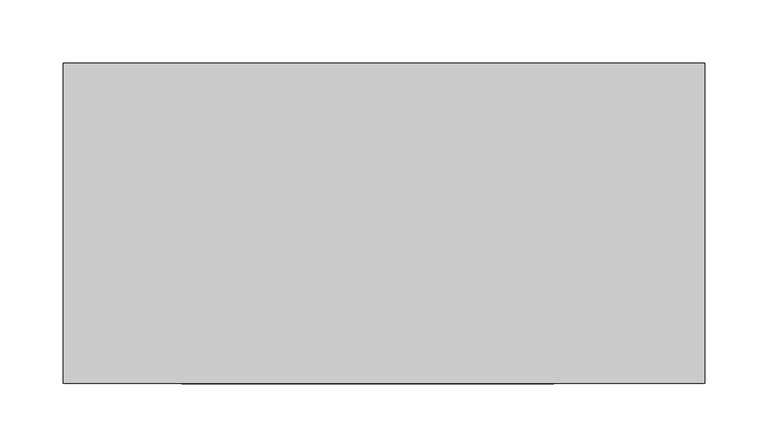
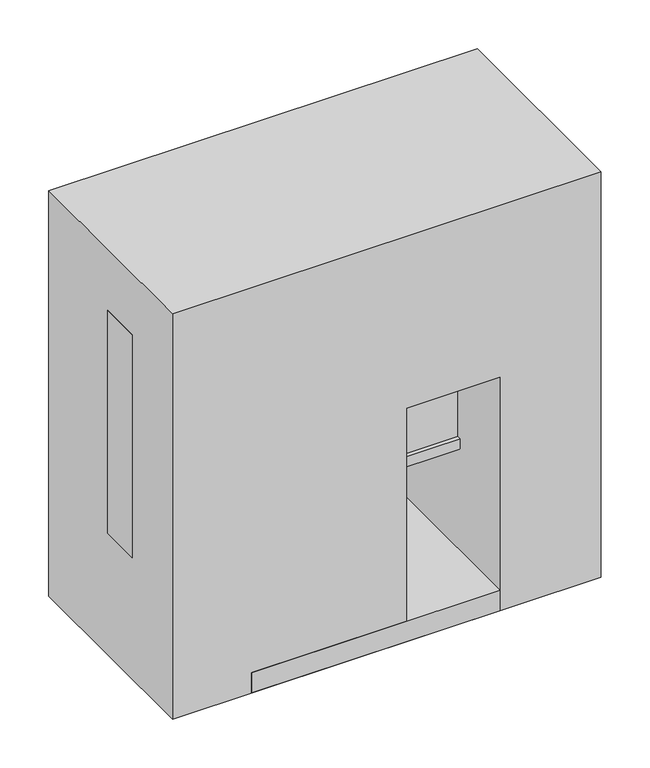
"""IFC4 building model written with IfcOpenShell, lengths in millimetres: proxy geometry, X4110 - Console, PACS, Remote View, 512 X 512, 1 Monitor : X4110 - Console, PACS, Remote View, 512 X 512, 1 Monitor."""

import ifcopenshell
import ifcopenshell.guid

model = None  # the IFC model being written
_history = None  # IfcOwnerHistory: only IFC2X3 demands one
_inside = {}  # id of a spatial element -> (the spatial element, [elements in it])
_under = {}  # id of a project, library or spatial element -> (it, [spatial elements below it])
_declared = {}  # id of a project -> (the project, [libraries it declares])
_typed = {}  # id of a type object -> (the type object, [elements of that type])
_made_of = {}  # id of a material, layer set ... -> (it, [elements and type objects made of it])


def new_model(schema):
    """Start an empty IFC model of exactly this schema.

    Asked for "IFC4X3", IfcOpenShell would pick the latest addendum, in which some entities
    have other attributes; the version numbers below select the first issue.
    IFC2X3 requires an IfcOwnerHistory on every rooted entity: one is made here for all.
    """
    global model, _history
    if schema == "IFC4X3":
        model = ifcopenshell.file(schema_version=(4, 3, 0, 0))
    else:
        model = ifcopenshell.file(schema=schema)
    _inside.clear()
    _under.clear()
    _declared.clear()
    _typed.clear()
    _made_of.clear()
    _history = None
    if model.schema == "IFC2X3":
        org = make("IfcOrganization", Name="unknown")
        user = make(
            "IfcPersonAndOrganization",
            ThePerson=make("IfcPerson", FamilyName="unknown"),
            TheOrganization=org,
        )
        app = make(
            "IfcApplication",
            ApplicationDeveloper=org,
            Version="unknown",
            ApplicationFullName="unknown",
            ApplicationIdentifier="unknown",
        )
        _history = make(
            "IfcOwnerHistory",
            OwningUser=user,
            OwningApplication=app,
            ChangeAction="ADDED",
            CreationDate=0,
        )
    return model


def make(cls, **values):
    """One entity of the class cls with the attributes given. An attribute that is None is left unset."""
    return model.create_entity(
        cls, **{name: value for name, value in values.items() if value is not None}
    )


def rooted(cls, **values):
    """An entity with a GlobalId (a new one), such as an element, a storey or a relation."""
    return make(cls, GlobalId=ifcopenshell.guid.new(), OwnerHistory=_history, **values)


def si_unit(unit_type, name, prefix=None):
    """IfcSIUnit, for example si_unit("LENGTHUNIT", "METRE", prefix="MILLI")."""
    return make("IfcSIUnit", UnitType=unit_type, Prefix=prefix, Name=name)


def assignment(units):
    """IfcUnitAssignment: the units of a project."""
    return None if units is None else make("IfcUnitAssignment", Units=units)


def point(xyz):
    """IfcCartesianPoint."""
    return None if xyz is None else make("IfcCartesianPoint", Coordinates=xyz)


def direction(xyz):
    """IfcDirection."""
    return None if xyz is None else make("IfcDirection", DirectionRatios=xyz)


def frame(location, z_axis=None, x_axis=None):
    """IfcAxis2Placement3D, a coordinate frame: its origin and axes. An axis left out is left unset."""
    return make(
        "IfcAxis2Placement3D",
        Location=point(location),
        Axis=direction(z_axis),
        RefDirection=direction(x_axis),
    )


def origin():
    """The frame at (0, 0, 0) with its axes left unset."""
    return frame((0.0, 0.0, 0.0))


def place(relative_to, where):
    """IfcLocalPlacement: puts the frame where relative to a parent placement (None: the world)."""
    return make(
        "IfcLocalPlacement", PlacementRelTo=relative_to, RelativePlacement=where
    )


def context(
    kind, dimensions, precision=None, world=None, true_north=None, identifier=None
):
    """IfcGeometricRepresentationContext, for example the 3D "Model" context."""
    return make(
        "IfcGeometricRepresentationContext",
        ContextIdentifier=identifier,
        ContextType=kind,
        CoordinateSpaceDimension=dimensions,
        Precision=precision,
        WorldCoordinateSystem=world,
        TrueNorth=true_north,
    )


def project(units=None, contexts=None):
    """IfcProject with its units and contexts."""
    return rooted(
        "IfcProject",
        Name="project",
        RepresentationContexts=contexts,
        UnitsInContext=assignment(units),
    )


def spatial(cls, under=None, at=None, **own):
    """A site, building, storey or space (cls), placed at a placement, below another one or the project."""
    s = rooted(cls, ObjectPlacement=at, **own)
    if under is not None:
        _under.setdefault(under.id(), (under, []))[1].append(s)
    return s


def faces_of(points, faces, orient=None, outer=None):
    """IfcFace entities. A face is a list of loops; a loop is a list of indices into points, from 0.

    orient and outer hold one flag for each loop. By default every Orientation is true, the
    first loop of a face is its IfcFaceOuterBound and the others are IfcFaceBound.
    """
    made = []
    for i, loops in enumerate(faces):
        bounds = []
        for j, loop in enumerate(loops):
            is_outer = j == 0 if outer is None else outer[i][j]
            bounds.append(
                make(
                    "IfcFaceOuterBound" if is_outer else "IfcFaceBound",
                    Bound=make("IfcPolyLoop", Polygon=[points[k] for k in loop]),
                    Orientation=True if orient is None else orient[i][j],
                )
            )
        made.append(make("IfcFace", Bounds=bounds))
    return made


def faceted_brep(points, faces, orient=None, outer=None, voids=None):
    """IfcFacetedBrep: a solid bounded by flat faces; with voids (closed shells), ...WithVoids."""
    shared = [point(p) for p in points]
    hull = make("IfcClosedShell", CfsFaces=faces_of(shared, faces, orient, outer))
    if voids is None:
        return make("IfcFacetedBrep", Outer=hull)
    return make(
        "IfcFacetedBrepWithVoids",
        Outer=hull,
        Voids=[
            make(cls, CfsFaces=faces_of(shared, fs, o, b)) for cls, fs, o, b in voids
        ],
    )


def shape(context_of_items, identifier, shape_type, items):
    """IfcShapeRepresentation: the items that make up one representation, for example the "Body"."""
    return make(
        "IfcShapeRepresentation",
        ContextOfItems=context_of_items,
        RepresentationIdentifier=identifier,
        RepresentationType=shape_type,
        Items=items,
    )


def source(mapping_origin, context_of_items, identifier, shape_type, items):
    """IfcRepresentationMap: a shape defined once, which mapped items show again and again."""
    return make(
        "IfcRepresentationMap",
        MappingOrigin=mapping_origin,
        MappedRepresentation=shape(context_of_items, identifier, shape_type, items),
    )


def transform(
    local_origin,
    x_axis=None,
    y_axis=None,
    z_axis=None,
    scale=None,
    scale2=None,
    scale3=None,
    uniform=True,
):
    """IfcCartesianTransformationOperator3D, or its non-uniform kind. x_axis, y_axis, z_axis: its Axis1, 2, 3."""
    if uniform:
        return make(
            "IfcCartesianTransformationOperator3D",
            Axis1=direction(x_axis),
            Axis2=direction(y_axis),
            LocalOrigin=point(local_origin),
            Scale=scale,
            Axis3=direction(z_axis),
        )
    return make(
        "IfcCartesianTransformationOperator3DnonUniform",
        Axis1=direction(x_axis),
        Axis2=direction(y_axis),
        LocalOrigin=point(local_origin),
        Scale=scale,
        Axis3=direction(z_axis),
        Scale2=scale2,
        Scale3=scale3,
    )


def mapped(mapping_source, mapping_target):
    """IfcMappedItem: shows the shape of a source again, moved by a transform."""
    return make(
        "IfcMappedItem", MappingSource=mapping_source, MappingTarget=mapping_target
    )


def made_of(thing, what):
    """Note that an element or type object is made of a material, layer set ...; save() writes the relation."""
    if what is not None:
        _made_of.setdefault(what.id(), (what, []))[1].append(thing)
    return thing


def element(
    cls,
    number,
    at=None,
    inside=None,
    cuts=None,
    type_object=None,
    material=None,
    context=None,
    identifier="Body",
    shape_type=None,
    held_by="IfcProductDefinitionShape",
    body=None,
    shapes=None,
    **own,
):
    """One element of the class cls, such as IfcWall. Its Tag is "e" and its number.

    at: its placement. inside: the storey or other place that contains it. cuts: it is an
    opening in that element (IfcRelVoidsElement). A single representation is given by context,
    identifier, shape_type and body (its items); several are given by shapes. held_by: the class
    of the entity that holds the representations. save() writes the other relations.
    """
    e = rooted(cls, Tag="e%d" % number, ObjectPlacement=at, **own)
    if body is not None:
        shapes = [shape(context, identifier, shape_type, body)]
    if shapes is not None:
        e.Representation = make(held_by, Representations=shapes)
    if inside is not None:
        _inside.setdefault(inside.id(), (inside, []))[1].append(e)
    if cuts is not None:
        rooted(
            "IfcRelVoidsElement", RelatingBuildingElement=cuts, RelatedOpeningElement=e
        )
    if type_object is not None:
        _typed.setdefault(type_object.id(), (type_object, []))[1].append(e)
    return made_of(e, material)


def aggregate(whole, parts):
    """IfcRelAggregates: a whole, such as a stair, and the parts it consists of."""
    return rooted("IfcRelAggregates", RelatingObject=whole, RelatedObjects=parts)


def save(model, path):
    """Write the relations noted so far, then the file.

    IfcRelAggregates (storeys below a building ...), IfcRelContainedInSpatialStructure (elements
    in a storey), IfcRelDefinesByType, IfcRelAssociatesMaterial and IfcRelDeclares: one each for
    every whole, place, type object, material and project.
    """
    for whole, parts in _under.values():
        aggregate(whole, parts)
    for where, things in _inside.values():
        rooted(
            "IfcRelContainedInSpatialStructure",
            RelatedElements=things,
            RelatingStructure=where,
        )
    for kind, things in _typed.values():
        rooted("IfcRelDefinesByType", RelatedObjects=things, RelatingType=kind)
    for what, things in _made_of.values():
        rooted("IfcRelAssociatesMaterial", RelatedObjects=things, RelatingMaterial=what)
    for by, libraries in _declared.values():
        rooted("IfcRelDeclares", RelatingContext=by, RelatedDefinitions=libraries)
    model.write(path)


def specialty_equipment_f5d2d7ad(model_context):
    return source(origin(), model_context, "Body", "Brep", [
        faceted_brep([(228.6, 6.2656905, 431.8), (-254.0, 6.2656905, 431.8), (-254.0, -44.3656905, 431.8), (228.6, -44.3656905, 431.8), (228.6, 6.2656905, 152.4), (228.6, -44.3656905, 152.4), (-254.0, -44.3656905, 152.4), (-254.0, 6.2656905, 152.4), (-241.3, -44.3656905, 419.1), (215.9, -44.3656905, 419.1), (215.9, -44.3656905, 165.1), (-241.3, -44.3656905, 165.1), (215.9, -39.5794881, 419.1), (-241.3, -39.5794881, 419.1), (215.9, -39.5794881, 165.1), (-241.3, -39.5794881, 165.1)], [[[0, 1, 2, 3]], [[4, 5, 6, 7]], [[1, 0, 4, 7]], [[2, 1, 7, 6]], [[3, 2, 6, 5], [8, 9, 10, 11]], [[0, 3, 5, 4]], [[12, 9, 8, 13]], [[14, 15, 11, 10]], [[12, 13, 15, 14]], [[13, 8, 11, 15]], [[9, 12, 14, 10]]]),
        faceted_brep([(134.5218395, -127.0, 25.4), (134.5218395, -127.0, 0.0), (134.5218395, 88.9, 0.0), (134.5218395, 88.9, 25.4), (-159.9218395, -127.0, 25.4), (-159.9218395, 88.9, 25.4), (-159.9218395, 88.9, 0.0), (-159.9218395, -127.0, 0.0), (24.2685686, 69.7656905, 31.75), (24.2685686, 69.7656905, 25.4), (-49.6685686, 69.7656905, 25.4), (-49.6685686, 69.7656905, 31.75), (24.2685686, 69.7656905, 292.1), (-49.6685686, 69.7656905, 292.1), (24.2685686, 6.2656905, 292.1), (-49.6685686, 6.2656905, 292.1), (24.2685686, 6.2656905, 241.3), (-49.6685686, 6.2656905, 241.3), (24.2685686, 44.3656905, 241.3), (-49.6685686, 44.3656905, 241.3), (24.2685686, 44.3656905, 25.4), (-49.6685686, 44.3656905, 25.4)], [[[0, 1, 2, 3]], [[4, 5, 6, 7]], [[8, 9, 10, 11]], [[12, 8, 11, 13]], [[14, 12, 13, 15]], [[16, 14, 15, 17]], [[18, 16, 17, 19]], [[20, 18, 19, 21]], [[0, 3, 5, 4], [20, 21, 10, 9]], [[1, 0, 4, 7]], [[2, 1, 7, 6]], [[5, 3, 2, 6]], [[20, 9, 8, 12, 14, 16, 18]], [[10, 21, 19, 17, 15, 13, 11]]]),
        faceted_brep([(254.0, 127.0, 508.0), (-254.0, 127.0, 508.0), (-254.0, -127.0, 508.0), (254.0, -127.0, 508.0), (254.0, 127.0, 0.0), (254.0, -127.0, 0.0), (-254.0, -127.0, 0.0), (-254.0, 127.0, 0.0), (24.2685686, -127.0, 292.1), (134.5218395, -127.0, 292.1), (134.5218395, -127.0, 25.4), (24.2685686, -127.0, 25.4), (134.5218395, 88.9, 292.1), (24.2685686, 88.9, 292.1), (24.2685686, 88.9, 25.4), (134.5218395, 88.9, 25.4)], [[[0, 1, 2, 3]], [[4, 5, 6, 7]], [[1, 0, 4, 7]], [[2, 1, 7, 6]], [[3, 2, 6, 5], [8, 9, 10, 11]], [[0, 3, 5, 4]], [[12, 13, 14, 15]], [[13, 12, 9, 8]], [[14, 13, 8, 11]], [[15, 14, 11, 10]], [[12, 15, 10, 9]]]),
    ])


if __name__ == "__main__":
    model = new_model("IFC4")
    model_context = context("Model", 3, world=origin())
    ifc_project = project(units=[si_unit("LENGTHUNIT", "METRE", prefix="MILLI")], contexts=[model_context])
    site = spatial("IfcSite", under=ifc_project)
    building = spatial("IfcBuilding", under=site)
    placement = place(None, origin())
    specialty_equipment_shape = specialty_equipment_f5d2d7ad(model_context)
    element("IfcBuildingElementProxy", 1, Name="X4110 - Console, PACS, Remote View, 512 X 512, 1 Monitor : X4110 - Console, PACS, Remote View, 512 X 512, 1 Monitor", ObjectType="X4110 - Console, PACS, Remote View, 512 X 512, 1 Monitor : X4110 - Console, PACS, Remote View, 512 X 512, 1 Monitor", at=placement, inside=building, context=model_context, shape_type="MappedRepresentation", body=[
        mapped(specialty_equipment_shape, transform((0.0, 0.0, 0.0), x_axis=(1.0, 0.0, 0.0), y_axis=(0.0, 1.0, 0.0), z_axis=(0.0, 0.0, 1.0))),
    ])
    save(model, "model.ifc")

# Revit data of these elements
# Type "X4110 - Console, PACS, Remote View, 512 X 512, 1 Monitor : X4110 - Console, PACS, Remote View, 512 X 512, 1 Monitor"
#   Watts2 = "0"
#   Watts1 = "240"
#   Unit_Issue = "EA"
#   UTIL_6_Misc = "-"
#   UTIL_5_NonMedGas = "-"
#   UTIL_4_MiscGas = "-"
#   UTIL_3_MedGas = "-"
#   UTIL_2_Elec = "B"
#   UTIL_1_WaterDrain = "-"
#   Nomenclature = "Console, PACS, Remote View, 512 X 512, 1 Monitor"
#   NSN = "6525"
#   Location [instance default] = ""
#   JSN = "X4110"
#   Fund_Source_VA = "-"
#   Fund_Source_Navy = "-"
#   Fund_Source_Army = "-"
#   Fund_Source_AF = "-"
#   ELEC_Volts2 = "0"
#   ELEC_Volts1 = "120"
#   ELEC_Phase2 = "0"
#   ELEC_Phase1 = "1"
#   ELEC_HertzSwitch = "0"
#   ELEC_HertzDependent = "0"
#   ELEC_Hertz = "50/60"
#   ELEC_Amps2 = "0"
#   ELEC_Amps1 = "2"
#   DetailDescription = "One monitor remote viewing station for picture archiving and retrieval (PACS) system. This station is for use by providers outside of radiology to review images and results. Station includes local image storage, image manipulation, and simultaneous display of multiple images on a single monitor. Images are stored on a resident hard disk and roll off the disk as more recent images are sent to the station by radiology. Provider may request images from the PACS. Unit must be connected to the PACS by LAN for image and result receipt. Console must be DICOM compliant. Input may be by keyboard, mouse, trackball or voice activated commands."
#   CAT_VA = "F"
#   CAT_Navy = "F"
#   CAT_IHS = "-"
#   CAT_Army = "F"
#   CAT_AF = "F"
#   BTUperhour = "0"
#   Weight_IP = 42
#   DIM_Width_IP = 1' - 8"
#   DIM_Height_IP = 1' - 8"
#   DIM_Depth_IP = 0' - 10"
#   finish [instance default] = none
#   Assembly Code = ""
# Element 1 (IfcBuildingElementProxy, "X4110 - Console, PACS, Remote View, 512 X 512, 1 Monitor : X4110 - Console, PACS, Remote View, 512 X 512, 1 Monitor")
#   Materials on its faces: "EquipSpace"
# Materials
#   "EquipSpace": class "Unassigned", colour RGB 221 217 195, transparency 0.5
